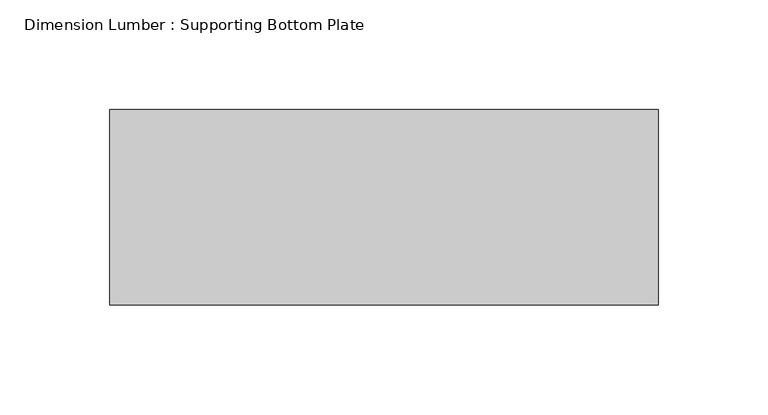
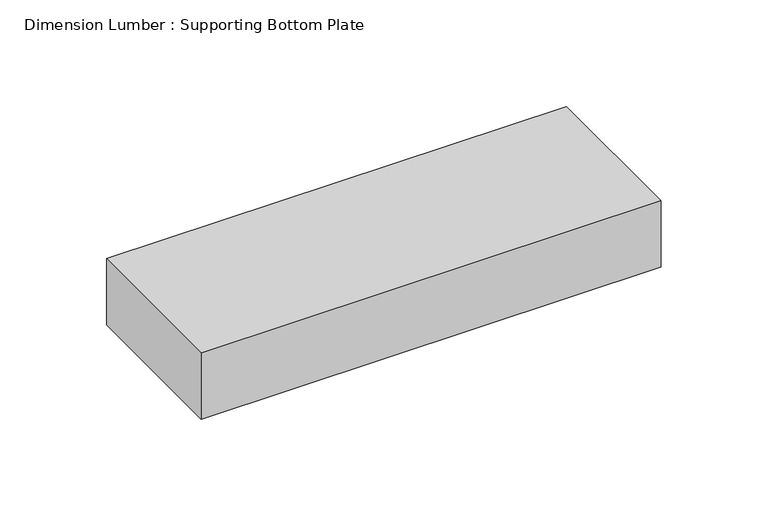
"""IFC4 building model written with IfcOpenShell, lengths in millimetres: beam geometry, Dimension Lumber : Supporting Bottom Plate."""

from ifc_helpers import new_model, si_unit, frame, origin, place, context, project, spatial, polyline, outline, extrude, source, transform, mapped, element, save


def dimension_lumber_supporting_bottom_plate_76e17ce6(model_context):
    return source(origin(), model_context, "Body", "SweptSolid", [
        extrude(outline(polyline([(146.8437503, 44.45), (146.8437503, -44.45), (-102.3937503, -44.45), (-102.3937503, 44.45), (146.8437503, 44.45)])), frame((0.0, 0.0, -19.05), z_axis=(0.0, 0.0, 1.0), x_axis=(1.0, 0.0, 0.0)), (0.0, 0.0, 1.0), 38.1),
    ])


if __name__ == "__main__":
    model = new_model("IFC4")
    model_context = context("Model", 3, world=origin())
    ifc_project = project(units=[si_unit("LENGTHUNIT", "METRE", prefix="MILLI")], contexts=[model_context])
    site = spatial("IfcSite", under=ifc_project)
    building = spatial("IfcBuilding", under=site)
    placement = place(None, origin())
    dimension_lumber_supporting_bottom_plate_shape = dimension_lumber_supporting_bottom_plate_76e17ce6(model_context)
    element("IfcBeam", 1, ObjectType="Dimension Lumber : Supporting Bottom Plate", at=placement, inside=building, context=model_context, shape_type="MappedRepresentation", body=[
        mapped(dimension_lumber_supporting_bottom_plate_shape, transform((0.0, 0.0, 0.0), x_axis=(1.0, 0.0, 0.0), y_axis=(0.0, 1.0, 0.0), z_axis=(0.0, 0.0, 1.0))),
    ])
    save(model, "model.ifc")

# Revit data of these elements
# Type "Dimension Lumber : Supporting Bottom Plate"
#   Assembly Code = "B10"
#   A = 0.0364583 SF
#   Length [instance default] = 5' - 0"
#   b = 0' - 3 1/2"
#   d = 0' - 1 1/2"
#   Structural Material [instance default] = Softwood, Lumber
# Element 1 (IfcBeam, "Dimension Lumber : Supporting Bottom Plate")
#   Structural Material = Douglas Fir #2
#   Materials on its faces: "Douglas Fir #2"
# Materials
#   "Softwood, Lumber": class "Wood", colour RGB 223 192 134, transparency 0, Description = "Pinus Echinata", Cost = 0
#   "Douglas Fir #2": class "Wood", colour RGB 223 192 134, transparency 0, Description = "Pinus Echinata", Cost = 0
